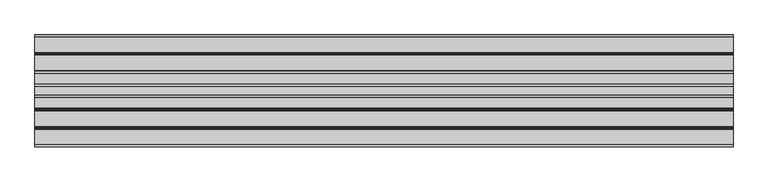
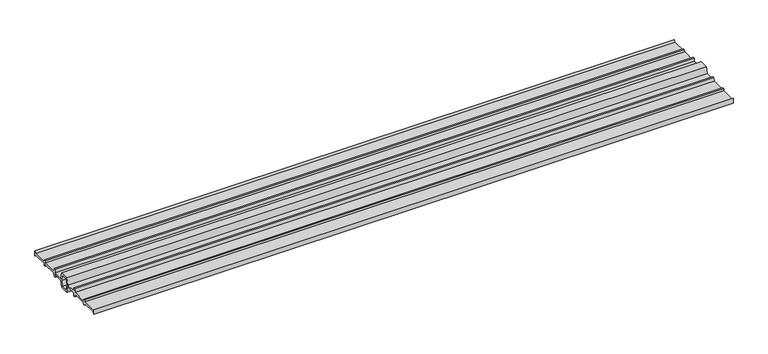
"""IFC4 building model written with IfcOpenShell, lengths in millimetres: proxy geometry, TN_ПВХ_ТПО_Гидрошпонка ТехноНИКОЛЬ : ПВХ Гидрошпонка ТехноНИКОЛЬ IM-240/20."""

from ifc_helpers import new_model, si_unit, frame, origin, place, context, project, spatial, polyline, outline, extrude, source, transform, mapped, element, save


def specialty_equipment_69b7e166(model_context):
    return source(origin(), model_context, "Body", "SweptSolid", [
        extrude(outline(polyline([(120.0, 8.0355304), (120.0, -3.7444008), (116.2555992, 0.0), (82.7344441, 0.0), (81.8662032, -4.9240388), (78.1337968, -4.9240388), (77.2655559, 0.0), (43.1139579, 0.0), (41.8418662, -7.7258715), (38.1581338, -7.7258715), (36.8860421, 0.0), (14.1057388, 0.0), (10.0, -15.3228258), (-10.0, -15.3228258), (-14.1057388, 0.0), (-36.8860421, 0.0), (-38.1581338, -7.7258715), (-41.8418662, -7.7258715), (-43.1139579, 0.0), (-77.2655559, 0.0), (-78.1337968, -4.9240388), (-81.8662032, -4.9240388), (-82.7344441, 0.0), (-116.2555992, 0.0), (-120.0, -3.7444008), (-120.0, 8.0355304), (-116.2555992, 4.2911296), (-82.6205653, 4.2911296), (-81.8662032, 8.8726426), (-78.1337968, 8.8726426), (-77.3794347, 4.2911296), (-43.1111586, 4.2911296), (-41.8418662, 12.0), (-38.1581338, 12.0), (-36.9722041, 4.7974211), (-14.1057388, 4.7974211), (-10.0, 20.1202469), (10.0, 20.1202469), (14.1057388, 4.7974211), (36.9722041, 4.7974211), (38.1581338, 12.0), (41.8418662, 12.0), (43.1111586, 4.2911296), (77.3804176, 4.2911296), (78.1337968, 8.8726426), (81.8662032, 8.8726426), (82.6205653, 4.2911296), (116.2555992, 4.2911296), (120.0, 8.0355304)]), holes=[polyline([(-9.5720905, 2.3987105), (-6.1633651, -10.3228258), (6.1633651, -10.3228258), (9.5720905, 2.3987105), (6.1633651, 15.1202469), (-6.1633651, 15.1202469), (-9.5720905, 2.3987105)])]), frame((0.0, 0.0, 0.0), z_axis=(1.0, 0.0, 0.0), x_axis=(0.0, 1.0, 0.0)), (0.0, 0.0, 1.0), 1500.0),
    ])


if __name__ == "__main__":
    model = new_model("IFC4")
    model_context = context("Model", 3, world=origin())
    ifc_project = project(units=[si_unit("LENGTHUNIT", "METRE", prefix="MILLI")], contexts=[model_context])
    site = spatial("IfcSite", under=ifc_project)
    building = spatial("IfcBuilding", under=site)
    placement = place(None, origin())
    specialty_equipment_shape = specialty_equipment_69b7e166(model_context)
    element("IfcBuildingElementProxy", 1, Name="TN_ПВХ_ТПО_Гидрошпонка ТехноНИКОЛЬ : ПВХ Гидрошпонка ТехноНИКОЛЬ IM-240/20", ObjectType="TN_ПВХ_ТПО_Гидрошпонка ТехноНИКОЛЬ : ПВХ Гидрошпонка ТехноНИКОЛЬ IM-240/20", at=placement, inside=building, context=model_context, shape_type="MappedRepresentation", body=[
        mapped(specialty_equipment_shape, transform((0.0, 0.0, 0.0), x_axis=(1.0, 0.0, 0.0), y_axis=(0.0, 1.0, 0.0), z_axis=(0.0, 0.0, 1.0))),
    ])
    save(model, "model.ifc")

# Revit data of these elements
# Type "TN_ПВХ_ТПО_Гидрошпонка ТехноНИКОЛЬ : ПВХ Гидрошпонка ТехноНИКОЛЬ IM-240/20"
#   Description = "Внутренняя деформационная ПВХ гидрошпонка. Применяется для герметизации деформационных швов при строительстве заглубленных и подземных сооружений. Ширина деформационного узла 20 мм."
#   Type Comments = "п.м."
#   Manufacturer = "ТехноНИКОЛЬ"
#   URL = "https://www.tn.ru/catalogue/dopolnitelnye_element2/gidroizoljacionnaja_shponka_tipa_vd_240/"
#   ADSK_Примечание = ""
#   ADSK_Обозначение [instance default] = "ТехноНИКОЛЬ"
#   ADSK_Наименование = "ПВХ Гидрошпонка ТехноНИКОЛЬ IM-240/20, 10м/рул"
#   ADSK_Масса_Текст = ""
#   ADSK_Марка = ""
#   ADSK_Код изделия = "499886"
#   ADSK_Завод-изготовитель [instance default] = "ТехноНИКОЛЬ"
#   ADSK_Единица измерения [instance default] = "п.м."
#   ADSK_Группирование = "Гидрошпонки"
#   ADSK_URL страницы изделия = "https://www.tn.ru/catalogue/dopolnitelnye_element2/gidroizoljacionnaja_shponka_tipa_vd_240/"
#   ADSK_URL документации изделия = "https://nav.tn.ru/upload/iblock/67f/Katalog-i-rekomendatsii-po-primeneniyu_Gidroshponki-TEKHNONIKOL.PDF"
#   built-in parameter 1001306 [instance default] = 3.28084 (stored number, unit not read)
#   ADSK_Размер_Длина [instance default] = 1000 mm
#   ADSK_Количество [instance default] = 1
#   ПВХ_ТПО Гидрошпонка ТехноНИКОЛЬ EC-320-4 = no
#   ПВХ Гидрошпонка ТехноНИКОЛЬ IM-260/50 = no
#   ПВХ Гидрошпонка ТехноНИКОЛЬ IM-240/20 = yes
#   ПВХ Гидрошпонка ТехноНИКОЛЬ IC-240-6 = no
#   ПВХ Гидрошпонка ТехноНИКОЛЬ IC-125-2SP = no
#   ПВХ Гидрошпонка ТехноНИКОЛЬ EM-260/50 = no
#   ПВХ Гидрошпонка ТехноНИКОЛЬ EM-260/20 = no
#   ПВХ Гидрошпонка ТехноНИКОЛЬ EC-320-4 = no
#   ПВХ Гидрошпонка ТехноНИКОЛЬ EC-220-3 = no
#   ПВХ_ТПО Гидрошпонка ТехноНИКОЛЬ EC-220-3 = no
#   ПВХ Гидрошпонка ТехноНИКОЛЬ IC-240-2 = no
#   Материал = TN_ПВХ_Черный
#   Default Elevation = 0
# Element 1 (IfcBuildingElementProxy, "TN_ПВХ_ТПО_Гидрошпонка ТехноНИКОЛЬ : ПВХ Гидрошпонка ТехноНИКОЛЬ IM-240/20")
#   built-in parameter 1001306 = 4.92126 (stored number, unit not read)
#   ADSK_Размер_Длина = 1500 mm
#   ADSK_Количество = 1.5
#   Materials on its faces: "TN_ПВХ_Черный"
# Materials
#   "TN_ПВХ_Черный": class "Типовые", colour RGB 48 48 48, transparency 0, Cost = 0
